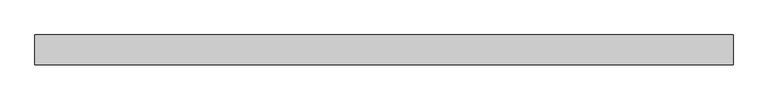
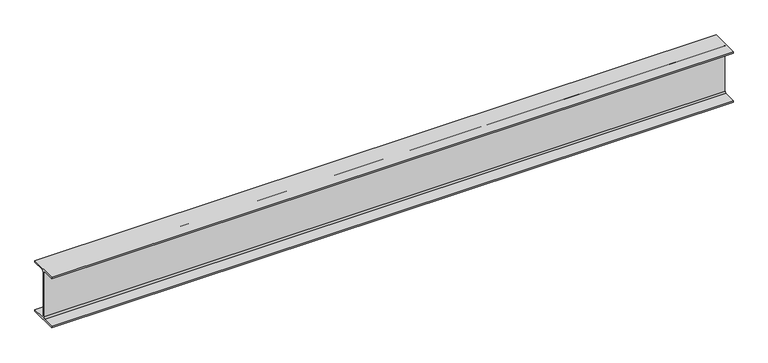
"""IFC4 building model written with IfcOpenShell, lengths in millimetres: beam geometry, Old_Steel Beam_H-KSD3502 : H_SB_ASB_H-250×125x6x9."""

from ifc_helpers import new_model, si_unit, point, frame, frame_2d, origin, place, context, project, spatial, polyline, circle_curve, trimmed, segment, composite_curve, outline, extrude, source, transform, mapped, element, save


def beam_8105422e(model_context):
    return source(origin(), model_context, "Body", "SweptSolid", [
        extrude(outline(composite_curve([segment(polyline([(82.5, -141.5), (82.5, -151.7), (-82.5, -151.7), (-82.5, -141.5), (-11.9, -141.5)]), True, "CONTINUOUS"), segment(trimmed(circle_curve(frame_2d((-11.9, -132.6)), 8.9), [point((-11.9, -141.5))], [point((-3.0, -132.6))], True, "CARTESIAN"), True, "CONTINUOUS"), segment(polyline([(-3.0, -132.6), (-3.0, 132.6)]), True, "CONTINUOUS"), segment(trimmed(circle_curve(frame_2d((-11.9, 132.6)), 8.9), [point((-3.0, 132.6))], [point((-11.9, 141.5))], True, "CARTESIAN"), True, "CONTINUOUS"), segment(polyline([(-11.9, 141.5), (-82.5, 141.5), (-82.5, 151.7), (82.5, 151.7), (82.5, 141.5), (11.9, 141.5)]), True, "CONTINUOUS"), segment(trimmed(circle_curve(frame_2d((11.9, 132.6)), 8.9), [point((11.9, 141.5))], [point((3.0, 132.6))], True, "CARTESIAN"), True, "CONTINUOUS"), segment(polyline([(3.0, 132.6), (3.0, -132.6)]), True, "CONTINUOUS"), segment(trimmed(circle_curve(frame_2d((11.9, -132.6)), 8.9), [point((3.0, -132.6))], [point((11.9, -141.5))], True, "CARTESIAN"), True, "CONTINUOUS"), segment(polyline([(11.9, -141.5), (82.5, -141.5)]), True, "CONTINUOUS")], self_intersect=False)), frame((-2029.8, 0.0, 0.0), z_axis=(1.0, 0.0, 0.0), x_axis=(0.0, 1.0, 0.0)), (0.0, 0.0, 1.0), 3859.8829189),
    ])


if __name__ == "__main__":
    model = new_model("IFC4")
    model_context = context("Model", 3, world=origin())
    ifc_project = project(units=[si_unit("LENGTHUNIT", "METRE", prefix="MILLI")], contexts=[model_context])
    site = spatial("IfcSite", under=ifc_project)
    building = spatial("IfcBuilding", under=site)
    placement = place(None, origin())
    beam_shape = beam_8105422e(model_context)
    element("IfcBeam", 1, ObjectType="Old_Steel Beam_H-KSD3502 : H_SB_ASB_H-250×125x6x9", at=placement, inside=building, context=model_context, shape_type="MappedRepresentation", body=[
        mapped(beam_shape, transform((0.0, 0.0, 0.0), x_axis=(1.0, 0.0, 0.0), y_axis=(0.0, 1.0, 0.0), z_axis=(0.0, 0.0, 1.0))),
    ])
    save(model, "model.ifc")

# Revit data of these elements
# Type "Old_Steel Beam_H-KSD3502 : H_SB_ASB_H-250×125x6x9"
#   Width = 12.5 cm
#   Web Thickness = 0.6 cm
#   Web Fillet = 1.2 cm
#   Warping Constant = 42539.8 cm⁶
#   Torsional Moment of Inertia = 7.8102 cm⁴
#   Torsional Modulus = 1.0 cm³
#   Section Area = 37.66 cm²
#   Plastic Modulus weak axis = 73.1 cm³
#   Plastic Modulus strong axis = 366.0 cm³
#   Perimeter = 0.97 m²/m
#   Nominal Weight = 29.60 kgf/m
#   Moment of Inertia weak axis = 294.00 cm⁴
#   Moment of Inertia strong axis = 4050.00 cm⁴
#   Height = 25.0 cm
#   Flange Thickness = 0.9 cm
#   Elastic Modulus weak axis = 47.0 cm³
#   Elastic Modulus strong axis = 324.0 cm³
#   Centroid Vertical = 12.5 cm
#   Centroid Horizontal = 6.25 cm
#   Length [instance default] = 1.5240 m
#   Structural Material [instance default] = Steel, 45-345
#   Assembly Code = ""
# Element 1 (IfcBeam, "Old_Steel Beam_H-KSD3502 : H_SB_ASB_H-250×125x6x9")
#   Structural Material = none
# Materials
#   "Steel, 45-345": class "Metal", colour RGB 189 187 185, transparency 0, Description = "Steel 345 MPa", Cost = 0
